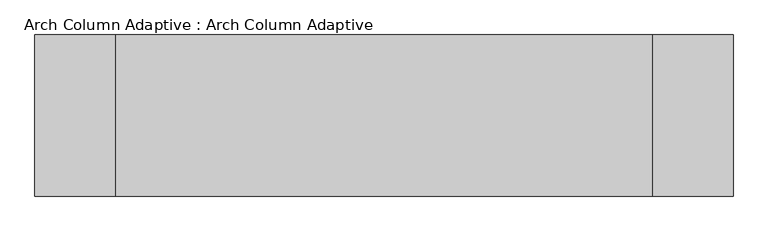
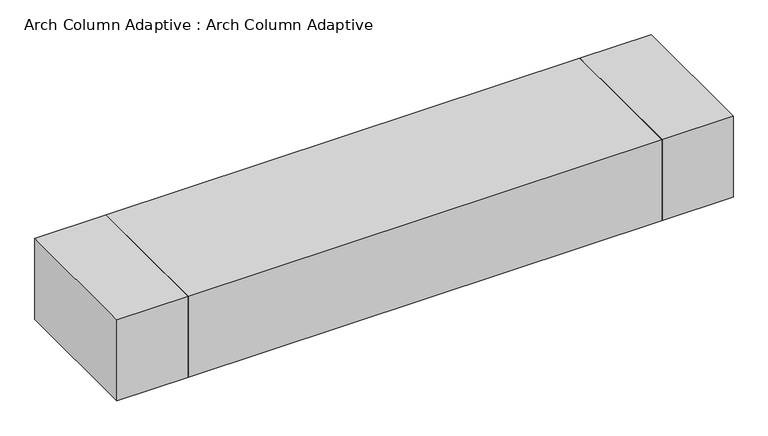
"""IFC4 building model written with IfcOpenShell, lengths in millimetres: proxy geometry, Arch Column Adaptive : Arch Column Adaptive."""

from ifc_helpers import new_model, si_unit, frame, origin, place, context, project, spatial, polyline, outline, extrude, source, transform, mapped, element, save


def arch_column_adaptive_arch_column_adaptive_5d259f20(model_context):
    return source(origin(), model_context, "Body", "SweptSolid", [
        extrude(outline(polyline([(5000.0, -1500.0), (5000.0, 1500.0), (6500.0, 1500.0), (6500.0, -1500.0), (5000.0, -1500.0)])), frame((0.0, 0.0, 46130.0), z_axis=(0.0, 0.0, 1.0), x_axis=(1.0, 0.0, 0.0)), (0.0, 0.0, 1.0), 1800.0),
        extrude(outline(polyline([(-5000.0, 1500.0), (-5000.0, -1500.0), (-6500.0, -1500.0), (-6500.0, 1500.0), (-5000.0, 1500.0)])), frame((0.0, 0.0, 46130.0), z_axis=(0.0, 0.0, 1.0), x_axis=(1.0, 0.0, 0.0)), (0.0, 0.0, 1.0), 1800.0),
        extrude(outline(polyline([(-5000.0, -1500.0), (-5000.0, 1500.0), (5000.0, 1500.0), (5000.0, -1500.0), (-5000.0, -1500.0)])), frame((0.0, 0.0, 46130.0), z_axis=(0.0, 0.0, 1.0), x_axis=(1.0, 0.0, 0.0)), (0.0, 0.0, 1.0), 1800.0),
    ])


if __name__ == "__main__":
    model = new_model("IFC4")
    model_context = context("Model", 3, world=origin())
    ifc_project = project(units=[si_unit("LENGTHUNIT", "METRE", prefix="MILLI")], contexts=[model_context])
    site = spatial("IfcSite", under=ifc_project)
    building = spatial("IfcBuilding", under=site)
    placement = place(None, origin())
    arch_column_adaptive_arch_column_adaptive_shape = arch_column_adaptive_arch_column_adaptive_5d259f20(model_context)
    element("IfcBuildingElementProxy", 1, Name="Arch Column Adaptive : Arch Column Adaptive", ObjectType="Arch Column Adaptive : Arch Column Adaptive", at=placement, inside=building, context=model_context, shape_type="MappedRepresentation", body=[
        mapped(arch_column_adaptive_arch_column_adaptive_shape, transform((0.0, 0.0, 0.0), x_axis=(1.0, 0.0, 0.0), y_axis=(0.0, 1.0, 0.0), z_axis=(0.0, 0.0, 1.0))),
    ])
    save(model, "model.ifc")

# Revit data of these elements
# Type "Arch Column Adaptive : Arch Column Adaptive"
#   Top Width = 3000 mm
#   Length [instance default] = 21000 mm
#   Height [instance default] = 50000 mm
#   Default Elevation = 0
# Element 1 (IfcBuildingElementProxy, "Arch Column Adaptive : Arch Column Adaptive")
#   Height = 46130 mm
